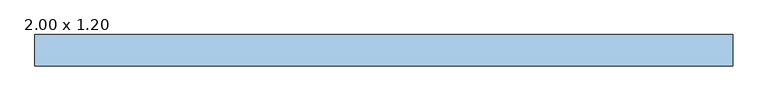
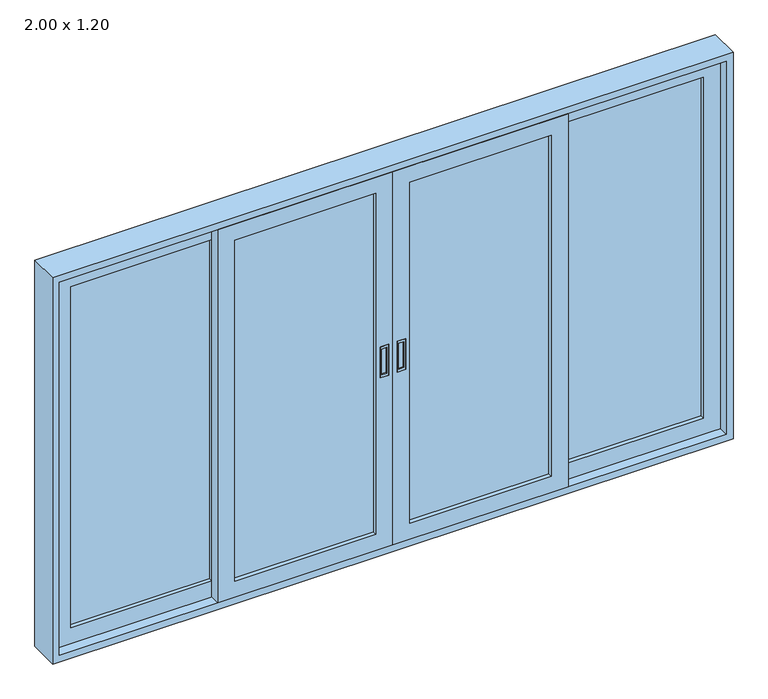
"""IFC4 building model written with IfcOpenShell, lengths in millimetres: window geometry, CC_JANELA CORRER_4 FOLHAS VIDRO : 2.00 x 1.20."""

import ifcopenshell
import ifcopenshell.guid

model = None  # the IFC model being written
_history = None  # IfcOwnerHistory: only IFC2X3 demands one
_inside = {}  # id of a spatial element -> (the spatial element, [elements in it])
_under = {}  # id of a project, library or spatial element -> (it, [spatial elements below it])
_declared = {}  # id of a project -> (the project, [libraries it declares])
_typed = {}  # id of a type object -> (the type object, [elements of that type])
_made_of = {}  # id of a material, layer set ... -> (it, [elements and type objects made of it])


def new_model(schema):
    """Start an empty IFC model of exactly this schema.

    Asked for "IFC4X3", IfcOpenShell would pick the latest addendum, in which some entities
    have other attributes; the version numbers below select the first issue.
    IFC2X3 requires an IfcOwnerHistory on every rooted entity: one is made here for all.
    """
    global model, _history
    if schema == "IFC4X3":
        model = ifcopenshell.file(schema_version=(4, 3, 0, 0))
    else:
        model = ifcopenshell.file(schema=schema)
    _inside.clear()
    _under.clear()
    _declared.clear()
    _typed.clear()
    _made_of.clear()
    _history = None
    if model.schema == "IFC2X3":
        org = make("IfcOrganization", Name="unknown")
        user = make(
            "IfcPersonAndOrganization",
            ThePerson=make("IfcPerson", FamilyName="unknown"),
            TheOrganization=org,
        )
        app = make(
            "IfcApplication",
            ApplicationDeveloper=org,
            Version="unknown",
            ApplicationFullName="unknown",
            ApplicationIdentifier="unknown",
        )
        _history = make(
            "IfcOwnerHistory",
            OwningUser=user,
            OwningApplication=app,
            ChangeAction="ADDED",
            CreationDate=0,
        )
    return model


def make(cls, **values):
    """One entity of the class cls with the attributes given. An attribute that is None is left unset."""
    return model.create_entity(
        cls, **{name: value for name, value in values.items() if value is not None}
    )


def rooted(cls, **values):
    """An entity with a GlobalId (a new one), such as an element, a storey or a relation."""
    return make(cls, GlobalId=ifcopenshell.guid.new(), OwnerHistory=_history, **values)


def si_unit(unit_type, name, prefix=None):
    """IfcSIUnit, for example si_unit("LENGTHUNIT", "METRE", prefix="MILLI")."""
    return make("IfcSIUnit", UnitType=unit_type, Prefix=prefix, Name=name)


def assignment(units):
    """IfcUnitAssignment: the units of a project."""
    return None if units is None else make("IfcUnitAssignment", Units=units)


def point(xyz):
    """IfcCartesianPoint."""
    return None if xyz is None else make("IfcCartesianPoint", Coordinates=xyz)


def direction(xyz):
    """IfcDirection."""
    return None if xyz is None else make("IfcDirection", DirectionRatios=xyz)


def frame(location, z_axis=None, x_axis=None):
    """IfcAxis2Placement3D, a coordinate frame: its origin and axes. An axis left out is left unset."""
    return make(
        "IfcAxis2Placement3D",
        Location=point(location),
        Axis=direction(z_axis),
        RefDirection=direction(x_axis),
    )


def origin():
    """The frame at (0, 0, 0) with its axes left unset."""
    return frame((0.0, 0.0, 0.0))


def place(relative_to, where):
    """IfcLocalPlacement: puts the frame where relative to a parent placement (None: the world)."""
    return make(
        "IfcLocalPlacement", PlacementRelTo=relative_to, RelativePlacement=where
    )


def context(
    kind, dimensions, precision=None, world=None, true_north=None, identifier=None
):
    """IfcGeometricRepresentationContext, for example the 3D "Model" context."""
    return make(
        "IfcGeometricRepresentationContext",
        ContextIdentifier=identifier,
        ContextType=kind,
        CoordinateSpaceDimension=dimensions,
        Precision=precision,
        WorldCoordinateSystem=world,
        TrueNorth=true_north,
    )


def project(units=None, contexts=None):
    """IfcProject with its units and contexts."""
    return rooted(
        "IfcProject",
        Name="project",
        RepresentationContexts=contexts,
        UnitsInContext=assignment(units),
    )


def spatial(cls, under=None, at=None, **own):
    """A site, building, storey or space (cls), placed at a placement, below another one or the project."""
    s = rooted(cls, ObjectPlacement=at, **own)
    if under is not None:
        _under.setdefault(under.id(), (under, []))[1].append(s)
    return s


def polyline(points):
    """IfcPolyline through the points."""
    return make("IfcPolyline", Points=[point(p) for p in points])


def outline(outer, holes=None, kind="AREA"):
    """IfcArbitraryClosedProfileDef: a profile drawn as a closed curve; with holes, ...WithVoids."""
    if holes is None:
        return make("IfcArbitraryClosedProfileDef", ProfileType=kind, OuterCurve=outer)
    return make(
        "IfcArbitraryProfileDefWithVoids",
        ProfileType=kind,
        OuterCurve=outer,
        InnerCurves=holes,
    )


def extrude(swept, where, along, depth):
    """IfcExtrudedAreaSolid: the profile swept, set in the frame where, extruded along a direction by depth."""
    return make(
        "IfcExtrudedAreaSolid",
        SweptArea=swept,
        Position=where,
        ExtrudedDirection=direction(along),
        Depth=depth,
    )


def faces_of(points, faces, orient=None, outer=None):
    """IfcFace entities. A face is a list of loops; a loop is a list of indices into points, from 0.

    orient and outer hold one flag for each loop. By default every Orientation is true, the
    first loop of a face is its IfcFaceOuterBound and the others are IfcFaceBound.
    """
    made = []
    for i, loops in enumerate(faces):
        bounds = []
        for j, loop in enumerate(loops):
            is_outer = j == 0 if outer is None else outer[i][j]
            bounds.append(
                make(
                    "IfcFaceOuterBound" if is_outer else "IfcFaceBound",
                    Bound=make("IfcPolyLoop", Polygon=[points[k] for k in loop]),
                    Orientation=True if orient is None else orient[i][j],
                )
            )
        made.append(make("IfcFace", Bounds=bounds))
    return made


def faceted_brep(points, faces, orient=None, outer=None, voids=None):
    """IfcFacetedBrep: a solid bounded by flat faces; with voids (closed shells), ...WithVoids."""
    shared = [point(p) for p in points]
    hull = make("IfcClosedShell", CfsFaces=faces_of(shared, faces, orient, outer))
    if voids is None:
        return make("IfcFacetedBrep", Outer=hull)
    return make(
        "IfcFacetedBrepWithVoids",
        Outer=hull,
        Voids=[
            make(cls, CfsFaces=faces_of(shared, fs, o, b)) for cls, fs, o, b in voids
        ],
    )


def shape(context_of_items, identifier, shape_type, items):
    """IfcShapeRepresentation: the items that make up one representation, for example the "Body"."""
    return make(
        "IfcShapeRepresentation",
        ContextOfItems=context_of_items,
        RepresentationIdentifier=identifier,
        RepresentationType=shape_type,
        Items=items,
    )


def source(mapping_origin, context_of_items, identifier, shape_type, items):
    """IfcRepresentationMap: a shape defined once, which mapped items show again and again."""
    return make(
        "IfcRepresentationMap",
        MappingOrigin=mapping_origin,
        MappedRepresentation=shape(context_of_items, identifier, shape_type, items),
    )


def transform(
    local_origin,
    x_axis=None,
    y_axis=None,
    z_axis=None,
    scale=None,
    scale2=None,
    scale3=None,
    uniform=True,
):
    """IfcCartesianTransformationOperator3D, or its non-uniform kind. x_axis, y_axis, z_axis: its Axis1, 2, 3."""
    if uniform:
        return make(
            "IfcCartesianTransformationOperator3D",
            Axis1=direction(x_axis),
            Axis2=direction(y_axis),
            LocalOrigin=point(local_origin),
            Scale=scale,
            Axis3=direction(z_axis),
        )
    return make(
        "IfcCartesianTransformationOperator3DnonUniform",
        Axis1=direction(x_axis),
        Axis2=direction(y_axis),
        LocalOrigin=point(local_origin),
        Scale=scale,
        Axis3=direction(z_axis),
        Scale2=scale2,
        Scale3=scale3,
    )


def mapped(mapping_source, mapping_target):
    """IfcMappedItem: shows the shape of a source again, moved by a transform."""
    return make(
        "IfcMappedItem", MappingSource=mapping_source, MappingTarget=mapping_target
    )


def made_of(thing, what):
    """Note that an element or type object is made of a material, layer set ...; save() writes the relation."""
    if what is not None:
        _made_of.setdefault(what.id(), (what, []))[1].append(thing)
    return thing


def element(
    cls,
    number,
    at=None,
    inside=None,
    cuts=None,
    type_object=None,
    material=None,
    context=None,
    identifier="Body",
    shape_type=None,
    held_by="IfcProductDefinitionShape",
    body=None,
    shapes=None,
    **own,
):
    """One element of the class cls, such as IfcWall. Its Tag is "e" and its number.

    at: its placement. inside: the storey or other place that contains it. cuts: it is an
    opening in that element (IfcRelVoidsElement). A single representation is given by context,
    identifier, shape_type and body (its items); several are given by shapes. held_by: the class
    of the entity that holds the representations. save() writes the other relations.
    """
    e = rooted(cls, Tag="e%d" % number, ObjectPlacement=at, **own)
    if body is not None:
        shapes = [shape(context, identifier, shape_type, body)]
    if shapes is not None:
        e.Representation = make(held_by, Representations=shapes)
    if inside is not None:
        _inside.setdefault(inside.id(), (inside, []))[1].append(e)
    if cuts is not None:
        rooted(
            "IfcRelVoidsElement", RelatingBuildingElement=cuts, RelatedOpeningElement=e
        )
    if type_object is not None:
        _typed.setdefault(type_object.id(), (type_object, []))[1].append(e)
    return made_of(e, material)


def aggregate(whole, parts):
    """IfcRelAggregates: a whole, such as a stair, and the parts it consists of."""
    return rooted("IfcRelAggregates", RelatingObject=whole, RelatedObjects=parts)


def save(model, path):
    """Write the relations noted so far, then the file.

    IfcRelAggregates (storeys below a building ...), IfcRelContainedInSpatialStructure (elements
    in a storey), IfcRelDefinesByType, IfcRelAssociatesMaterial and IfcRelDeclares: one each for
    every whole, place, type object, material and project.
    """
    for whole, parts in _under.values():
        aggregate(whole, parts)
    for where, things in _inside.values():
        rooted(
            "IfcRelContainedInSpatialStructure",
            RelatedElements=things,
            RelatingStructure=where,
        )
    for kind, things in _typed.values():
        rooted("IfcRelDefinesByType", RelatedObjects=things, RelatingType=kind)
    for what, things in _made_of.values():
        rooted("IfcRelAssociatesMaterial", RelatedObjects=things, RelatingMaterial=what)
    for by, libraries in _declared.values():
        rooted("IfcRelDeclares", RelatingContext=by, RelatedDefinitions=libraries)
    model.write(path)


def window_2_00_x_1_20_63c3f2e4(model_context):
    return source(origin(), model_context, "Body", "SolidModel", [
        extrude(outline(polyline([(17.5, -96.0), (17.5, -95.0), (32.5, -95.0), (32.5, -96.0), (17.5, -96.0)])), frame((0.0, 0.0, 1560.0), z_axis=(0.0, 0.0, 1.0), x_axis=(1.0, 0.0, 0.0)), (0.0, 0.0, 1.0), 80.0),
        extrude(outline(polyline([(1552.0, 37.5), (1648.0, 37.5), (1648.0, 12.5), (1552.0, 12.5), (1552.0, 37.5)]), holes=[polyline([(1560.0, 32.5), (1560.0, 17.5), (1640.0, 17.5), (1640.0, 32.5), (1560.0, 32.5)])]), frame((0.0, -100.1, 0.0), z_axis=(0.0, 1.0, 0.0), x_axis=(0.0, 0.0, 1.0)), (0.0, 0.0, 1.0), 5.1),
        faceted_brep([(50.0, -100.0, 2130.0), (50.0, -100.0, 1070.0), (50.0, -70.0, 1070.0), (50.0, -70.0, 2130.0), (0.0, -70.0, 2180.0), (515.0, -70.0, 2180.0), (515.0, -70.0, 1020.0), (0.0, -70.0, 1020.0), (465.0, -70.0, 1070.0), (465.0, -70.0, 2130.0), (465.0, -100.0, 1070.0), (0.0, -100.0, 1020.0), (515.0, -100.0, 1020.0), (515.0, -100.0, 2180.0), (0.0, -100.0, 2180.0), (37.5, -100.0, 1648.0), (37.5, -100.0, 1552.0), (12.5, -100.0, 1552.0), (12.5, -100.0, 1648.0), (465.0, -100.0, 2130.0), (12.5, -95.0, 1552.0), (12.5, -95.0, 1648.0), (37.5, -95.0, 1552.0), (37.5, -95.0, 1648.0)], [[[0, 1, 2, 3]], [[4, 5, 6, 7], [2, 8, 9, 3]], [[1, 10, 8, 2]], [[11, 12, 13, 14], [15, 16, 17, 18], [0, 19, 10, 1]], [[4, 7, 11, 14]], [[7, 6, 12, 11]], [[10, 19, 9, 8]], [[6, 5, 13, 12]], [[18, 17, 20, 21]], [[20, 17, 16, 22]], [[23, 22, 16, 15]], [[21, 20, 22, 23]], [[3, 9, 19, 0]], [[14, 13, 5, 4]], [[21, 23, 15, 18]]]),
        extrude(outline(polyline([(50.0, -82.5), (465.0, -82.5), (465.0, -87.5), (50.0, -87.5), (50.0, -82.5)])), frame((0.0, 0.0, 1070.0), z_axis=(0.0, 0.0, 1.0), x_axis=(1.0, 0.0, 0.0)), (0.0, 0.0, 1.0), 1060.0),
        extrude(outline(polyline([(-17.5, -96.0), (-32.5, -96.0), (-32.5, -95.0), (-17.5, -95.0), (-17.5, -96.0)])), frame((0.0, 0.0, 1560.0), z_axis=(0.0, 0.0, 1.0), x_axis=(1.0, 0.0, 0.0)), (0.0, 0.0, 1.0), 80.0),
        extrude(outline(polyline([(1552.0, -37.5), (1552.0, -12.5), (1648.0, -12.5), (1648.0, -37.5), (1552.0, -37.5)]), holes=[polyline([(1560.0, -32.5), (1640.0, -32.5), (1640.0, -17.5), (1560.0, -17.5), (1560.0, -32.5)])]), frame((0.0, -100.1, 0.0), z_axis=(0.0, 1.0, 0.0), x_axis=(0.0, 0.0, 1.0)), (0.0, 0.0, 1.0), 5.1),
        faceted_brep([(-50.0, -100.0, 2130.0), (-50.0, -70.0, 2130.0), (-50.0, -70.0, 1070.0), (-50.0, -100.0, 1070.0), (0.0, -70.0, 2180.0), (0.0, -70.0, 1020.0), (-515.0, -70.0, 1020.0), (-515.0, -70.0, 2180.0), (-465.0, -70.0, 2130.0), (-465.0, -70.0, 1070.0), (-465.0, -100.0, 1070.0), (0.0, -100.0, 1020.0), (0.0, -100.0, 2180.0), (-515.0, -100.0, 2180.0), (-515.0, -100.0, 1020.0), (-465.0, -100.0, 2130.0), (-37.5, -100.0, 1648.0), (-12.5, -100.0, 1648.0), (-12.5, -100.0, 1552.0), (-37.5, -100.0, 1552.0), (-12.5, -95.0, 1648.0), (-12.5, -95.0, 1552.0), (-37.5, -95.0, 1552.0), (-37.5, -95.0, 1648.0)], [[[0, 1, 2, 3]], [[4, 5, 6, 7], [2, 1, 8, 9]], [[3, 2, 9, 10]], [[11, 12, 13, 14], [0, 3, 10, 15], [16, 17, 18, 19]], [[4, 12, 11, 5]], [[5, 11, 14, 6]], [[10, 9, 8, 15]], [[6, 14, 13, 7]], [[17, 20, 21, 18]], [[21, 22, 19, 18]], [[23, 16, 19, 22]], [[20, 23, 22, 21]], [[1, 0, 15, 8]], [[12, 4, 7, 13]], [[20, 17, 16, 23]]]),
        extrude(outline(polyline([(-50.0, -82.5), (-50.0, -87.5), (-465.0, -87.5), (-465.0, -82.5), (-50.0, -82.5)])), frame((0.0, 0.0, 1070.0), z_axis=(0.0, 0.0, 1.0), x_axis=(1.0, 0.0, 0.0)), (0.0, 0.0, 1.0), 1060.0),
        extrude(outline(polyline([(930.0, -52.5), (930.0, -57.5), (515.0, -57.5), (515.0, -52.5), (930.0, -52.5)])), frame((0.0, 0.0, 1070.0), z_axis=(0.0, 0.0, 1.0), x_axis=(1.0, 0.0, 0.0)), (0.0, 0.0, 1.0), 1060.0),
        extrude(outline(polyline([(2180.0, 980.0), (2180.0, 465.0), (1020.0, 465.0), (1020.0, 980.0), (2180.0, 980.0)]), holes=[polyline([(1070.0, 930.0), (1070.0, 515.0), (2130.0, 515.0), (2130.0, 930.0), (1070.0, 930.0)])]), frame((0.0, -70.0, 0.0), z_axis=(0.0, 1.0, 0.0), x_axis=(0.0, 0.0, 1.0)), (0.0, 0.0, 1.0), 30.0),
        extrude(outline(polyline([(-515.0, -52.5), (-515.0, -57.5), (-930.0, -57.5), (-930.0, -52.5), (-515.0, -52.5)])), frame((0.0, 0.0, 1070.0), z_axis=(0.0, 0.0, 1.0), x_axis=(1.0, 0.0, 0.0)), (0.0, 0.0, 1.0), 1060.0),
        extrude(outline(polyline([(2180.0, -465.0), (2180.0, -980.0), (1020.0, -980.0), (1020.0, -465.0), (2180.0, -465.0)]), holes=[polyline([(1070.0, -515.0), (1070.0, -930.0), (2130.0, -930.0), (2130.0, -515.0), (1070.0, -515.0)])]), frame((0.0, -70.0, 0.0), z_axis=(0.0, 1.0, 0.0), x_axis=(0.0, 0.0, 1.0)), (0.0, 0.0, 1.0), 30.0),
        extrude(outline(polyline([(2200.0, 1000.0), (2200.0, -1000.0), (1000.0, -1000.0), (1000.0, 1000.0), (2200.0, 1000.0)]), holes=[polyline([(2180.0, 980.0), (1020.0, 980.0), (1020.0, -980.0), (2180.0, -980.0), (2180.0, 980.0)])]), frame((0.0, -100.0, 0.0), z_axis=(0.0, 1.0, 0.0), x_axis=(0.0, 0.0, 1.0)), (0.0, 0.0, 1.0), 90.0),
    ])


if __name__ == "__main__":
    model = new_model("IFC4")
    model_context = context("Model", 3, world=origin())
    ifc_project = project(units=[si_unit("LENGTHUNIT", "METRE", prefix="MILLI")], contexts=[model_context])
    site = spatial("IfcSite", under=ifc_project)
    building = spatial("IfcBuilding", under=site)
    placement = place(None, origin())
    window_2_00_x_1_20_shape = window_2_00_x_1_20_63c3f2e4(model_context)
    element("IfcWindow", 1, ObjectType="CC_JANELA CORRER_4 FOLHAS VIDRO : 2.00 x 1.20", at=placement, inside=building, context=model_context, shape_type="MappedRepresentation", body=[
        mapped(window_2_00_x_1_20_shape, transform((0.0, 0.0, 0.0), x_axis=(1.0, 0.0, 0.0), y_axis=(0.0, 1.0, 0.0), z_axis=(0.0, 0.0, 1.0))),
    ])
    save(model, "model.ifc")

# Revit data of these elements
# Type "CC_JANELA CORRER_4 FOLHAS VIDRO : 2.00 x 1.20"
#   Type Mark = "J7"
#   Site = "www.construir.arq.br"
#   Emprea = "Cursos Construir"
#   Criado Por = "Roberto Netto"
#   Analytic Construction = "<Nenhum>"
#   Rough Width = 2.00 m
#   Largura Moldura Folha [instance default] = 0.05 m
#   Largura Guarnição Interna [instance default] = 0.10 m
#   Largura Moldura Externa [instance default] = 0.10 m
#   Largura Folha [instance default] = 0.515 m
#   Interna [instance default] = 0.00 m
#   Externa [instance default] = 0.00 m
#   Extensão Frontal Peitoril/Pingadeira [instance default] = 0.03 m
#   Extensão Exterior Esquerda Peitoril/Pingadeira [instance default] = 0.025 m
#   Extensão Exterior Direita Peitoril/Pingadeira [instance default] = 0.025 m
#   Extensão Caixilho [instance default] = 0.03 m
#   Espessura Peitoril/Pingadeira [instance default] = 0.02 m
#   Espessura Guarnição Interna [instance default] = 0.005 m
#   Espessura Moldura Externa [instance default] = 0.01 m
#   Espessura Folha [instance default] = 0.03 m
#   Cálculo Porcentagem [instance default] = 0.00 m
#   Cálculo Abertura [instance default] = 0.00 m
#   Espessura Caixilho [instance default] = 0.02 m
#   Rough Height = 1.20 m
#   Altura Folha [instance default] = 1.16 m
#   Altura Corte [instance default] = 0.02 m
#   Height = 1.20 m
#   Width = 2.00 m
#   ----PEITORIL/PINGADEIRA--- [instance default] = 0.00 m
#   ----MOLDURA---- [instance default] = 0.00 m
#   ----GUARNIÇÃO---- [instance default] = 0.00 m
#   ----EXTENSÃO---- [instance default] = 0.00 m
#   ----CAIXILHO---- [instance default] = 0.00 m
#   -----FOLHA---- [instance default] = 0.00 m
#   Puxador [instance default] = yes
#   Peitoril/Pingadeira Vazio [instance default] = no
#   Peitoril/Pingadeira Família [instance default] = yes
#   Guarnição Interna [instance default] = yes
#   Moldura Externa Sem Peitoril [instance default] = no
#   Moldura Externa Com Peitoril [instance default] = yes
#   Moldura Externa [instance default] = yes
#   Material Vidro Folha = .VIDRO
#   Material Puxador = .ALUMÍNIO COM PINTURA ELETROSTÁTICA BRANCA
#   Material Peitoril/Pingadeira = .GRANITO BRANCO ITAÚNAS
#   Material Moldura Folha = .ALUMÍNIO COM PINTURA ELETROSTÁTICA BRANCA
#   Material Moldura Externa = .PINTURA ACRÍLICA BRANCA
#   Material Caixilho = .ALUMÍNIO COM PINTURA ELETROSTÁTICA BRANCA
#   Material Guarnição = .ALUMÍNIO COM PINTURA ELETROSTÁTICA BRANCA
#   Wall Closure = (empty or 0)
# Element 1 (IfcWindow, "CC_JANELA CORRER_4 FOLHAS VIDRO : 2.00 x 1.20")
#   Guarnição Interna = no
#   Moldura Externa Com Peitoril = no
#   Moldura Externa = no
#   Materials on its faces: ".ALUMÍNIO COM PINTURA ELETROSTÁTICA BRANCA", ".VIDRO"
# Materials
#   ".VIDRO": class "Genérico", colour RGB 198 236 255, transparency 0.95, Cost = 0
#   ".ALUMÍNIO COM PINTURA ELETROSTÁTICA BRANCA": class "CC_METAIS", colour RGB 241 241 241, transparency 0, Cost = 0
#   ".GRANITO BRANCO ITAÚNAS": class ".CC_PEDRA REVEST.", colour RGB 202 195 174, transparency 0, Description = "Granito branco Itaúnas", Uso = "Pedra", Cost = 0
#   ".PINTURA ACRÍLICA BRANCA": class ".CC_PINTURA", colour RGB 250 250 250, transparency 0, Keynote = "09910.A1", Description = "Tinta acrílica na cor branca", Uso = "Pint.", Cost = 0
